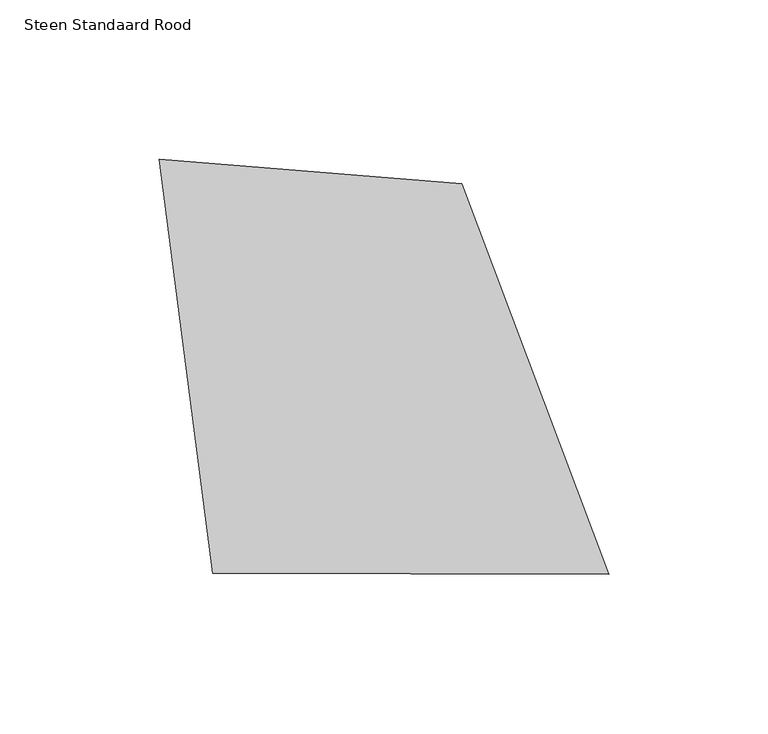
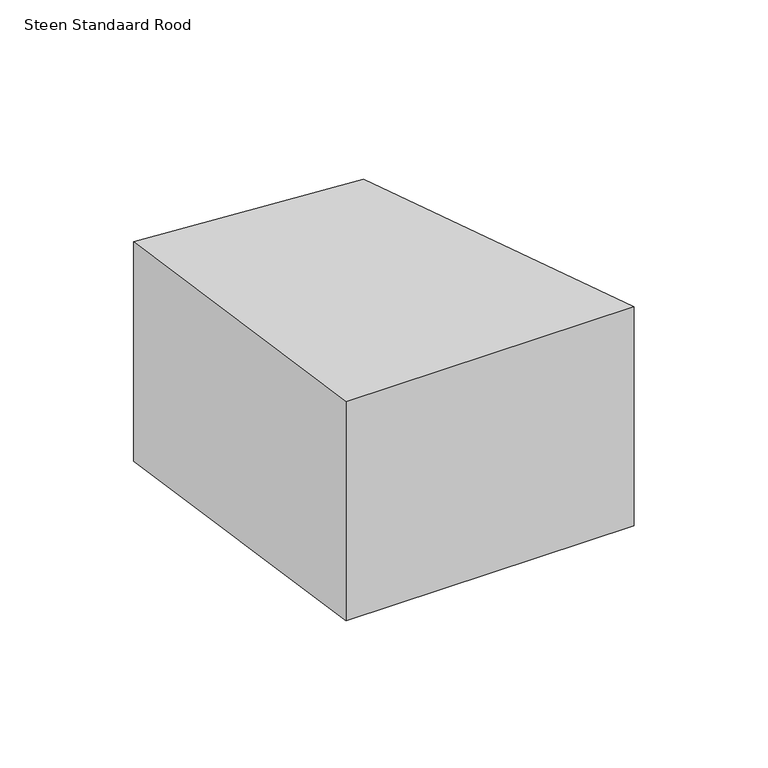
"""IFC4 building model written with IfcOpenShell, lengths in millimetres: proxy geometry, 00_GMA_steen_versie_4 : Steen Standaard Rood."""

from ifc_helpers import new_model, si_unit, origin, origin_with_axes, place, context, project, spatial, polyline, outline, extrude, source, transform, mapped, element, save


def steen_standaard_rood_a5b9f397(model_context):
    return source(origin(), model_context, "Body", "SweptSolid", [
        extrude(outline(polyline([(82.4636514, 127.1543377), (128.4615135, 4.6891223), (4.3616271, 4.9486265), (-12.4180967, 134.7857038), (82.4636514, 127.1543377)])), origin_with_axes(), (0.0, 0.0, 1.0), 100.0),
    ])


if __name__ == "__main__":
    model = new_model("IFC4")
    model_context = context("Model", 3, world=origin())
    ifc_project = project(units=[si_unit("LENGTHUNIT", "METRE", prefix="MILLI")], contexts=[model_context])
    site = spatial("IfcSite", under=ifc_project)
    building = spatial("IfcBuilding", under=site)
    placement = place(None, origin())
    steen_standaard_rood_shape = steen_standaard_rood_a5b9f397(model_context)
    element("IfcBuildingElementProxy", 1, Name="00_GMA_steen_versie_4 : Steen Standaard Rood", ObjectType="00_GMA_steen_versie_4 : Steen Standaard Rood", at=placement, inside=building, context=model_context, shape_type="MappedRepresentation", body=[
        mapped(steen_standaard_rood_shape, transform((0.0, 0.0, 0.0), x_axis=(1.0, 0.0, 0.0), y_axis=(0.0, 1.0, 0.0), z_axis=(0.0, 0.0, 1.0))),
    ])
    save(model, "model.ifc")

# Revit data of these elements
# Type "00_GMA_steen_versie_4 : Steen Standaard Rood"
#   StootVoegHalfBoven [instance default] = 5 mm
#   StootVoegHalf [instance default] = 5 mm
#   StootVoegBreedteOnder = 10 mm
#   StootVoegBreedteBoven = 10 mm
#   Steendikte = 100 mm
#   LintVoegOnderHalf = 5 mm
#   LintVoegOnder = 10 mm
#   LintVoegBovenHalf = 5 mm
#   LintVoegBoven = 10 mm
#   materiaal = 21_steen_rood
#   MateriaalVoeg = none
#   Default Elevation = 0
# Element 1 (IfcBuildingElementProxy, "00_GMA_steen_versie_4 : Steen Standaard Rood")
#   Materials on its faces: "21_steen_rood"
# Materials
#   "21_steen_rood": class "Unassigned", colour RGB 213 111 43, transparency 0, Cost = 0
